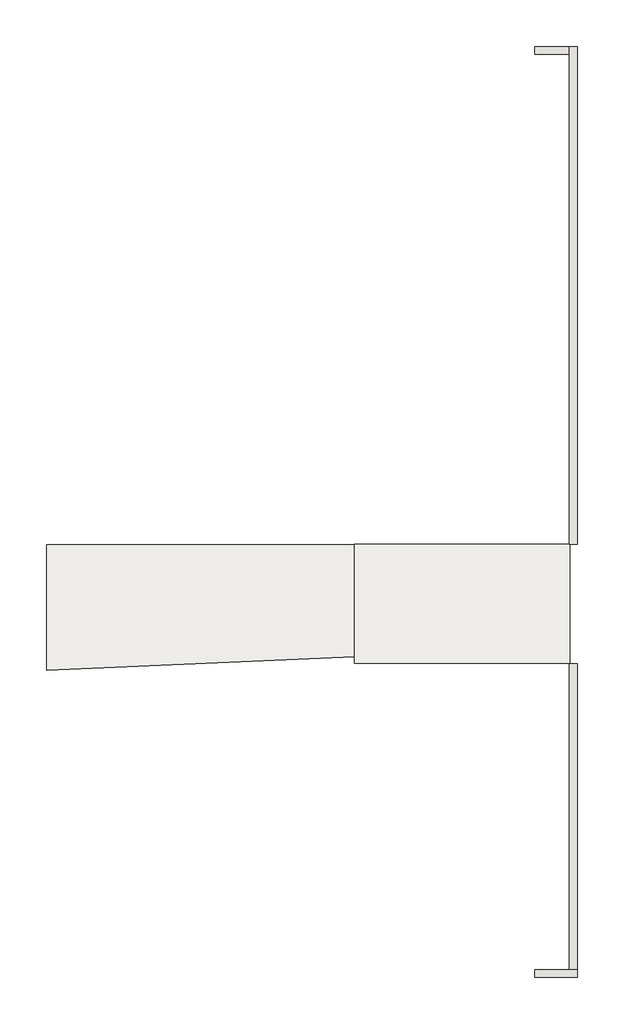
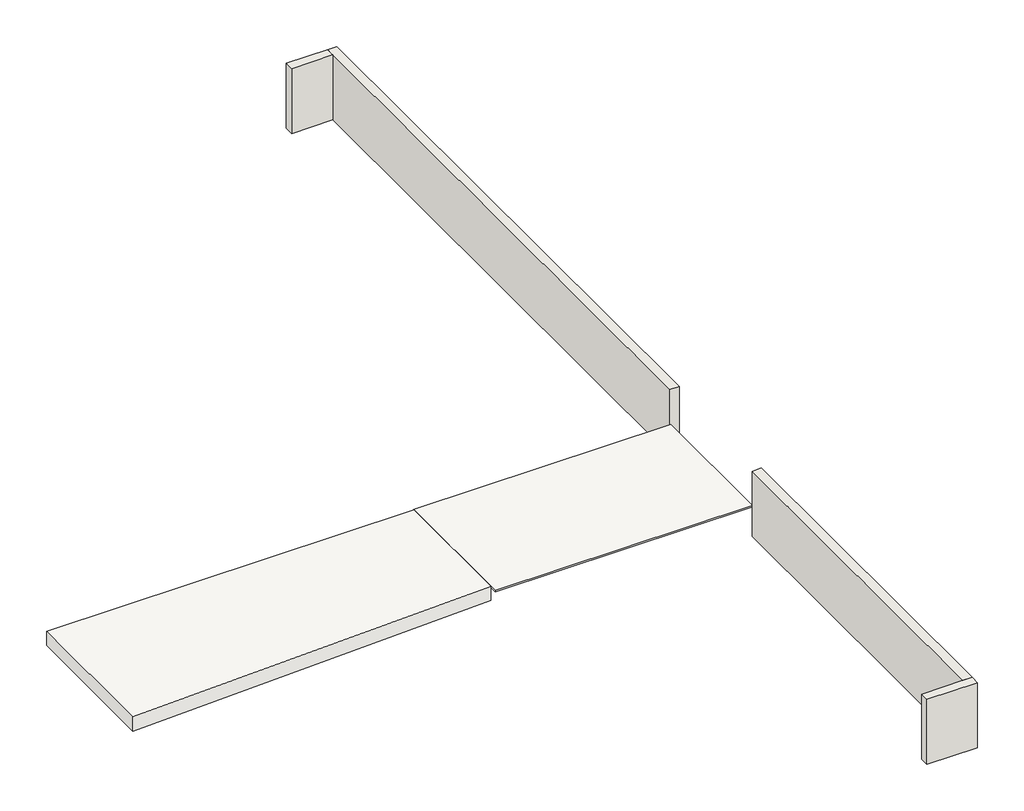
# One storey: 4 walls, 2 slabs.
"""IFC4 building model written with IfcOpenShell, lengths in millimetres."""

from ifc_helpers import new_model, si_unit, frame, origin, place, context, project, spatial, polyline, outline, extrude, faceted_brep, element, save

model = new_model("IFC4")

# Units and contexts
model_context = context("Model", 3, world=origin())
ifc_project = project(units=[si_unit("LENGTHUNIT", "METRE", prefix="MILLI")], contexts=[model_context])

# Site, building, storey
site = spatial("IfcSite", under=ifc_project)
building = spatial("IfcBuilding", under=site)
storey = spatial("IfcBuildingStorey", under=building, Name="otopark", Elevation=-660.0)

# Slabs
placement = place(None, origin())
element("IfcSlab", 1, ObjectType="aa Taban 3 cm beyaz mermer", at=placement, inside=storey, context=model_context, shape_type="SweptSolid", body=[
    extrude(outline(polyline([(11307.8247381, -10362.4985309), (11307.8247381, -7282.4985309), (16907.8247381, -7282.4985309), (16907.8247381, -10362.4985309), (11307.8247381, -10362.4985309)])), frame((0.0, 0.0, -689.8), z_axis=(0.0, 0.0, 1.0), x_axis=(1.0, 0.0, 0.0)), (0.0, 0.0, 1.0), 30.0),
])
element("IfcSlab", 2, ObjectType="15mm Foundation Slab", at=placement, inside=storey, context=model_context, shape_type="Brep", body=[
    faceted_brep([(11307.8247381, -7292.4985309, -989.8), (11307.8247381, -10202.8108149, -989.8), (3307.8247381, -10546.9586554, -989.8), (3307.8247381, -7292.4985309, -989.8), (11307.8247381, -7292.4985309, -659.8), (3307.8247381, -7292.4985309, -659.8), (3307.8247381, -10546.9586554, -659.8), (11307.8247381, -10202.8108149, -659.8), (3307.8247381, -7292.4985309, -930.0)], [[[0, 1, 2, 3]], [[4, 5, 6, 7]], [[1, 0, 4, 7]], [[2, 1, 7, 6]], [[3, 2, 6, 5, 8]], [[0, 3, 8, 5, 4]]]),
])

# Walls
element("IfcWall", 3, ObjectType="Generic - 200mm - Filled", at=placement, inside=storey, context=model_context, shape_type="SweptSolid", body=[
    extrude(outline(polyline([(17100.9898032, -10378.1142076), (17100.9898032, -18328.1142076), (16900.9898032, -18328.1142076), (16900.9898032, -10378.1142076), (17100.9898032, -10378.1142076)])), frame((0.0, 0.0, -1360.0), z_axis=(0.0, 0.0, 1.0), x_axis=(1.0, 0.0, 0.0)), (0.0, 0.0, 1.0), 1500.0),
])
element("IfcWall", 4, ObjectType="Generic - 200mm - Filled", at=placement, inside=storey, context=model_context, shape_type="Brep", body=[
    faceted_brep([(17100.9898032, -7272.9665452, -1360.0), (17100.9898032, 5647.0334548, -1360.0), (17100.9898032, 5647.0334548, 140.0), (17100.9898032, -7272.9665452, 140.0), (16900.9898032, -7272.9665452, -1360.0), (16900.9898032, -7272.9665452, 140.0), (16900.9898032, 5447.0334548, 140.0), (16900.9898032, 5647.0334548, 140.0), (16900.9898032, 5647.0334548, -1360.0), (16900.9898032, 5447.0334548, -1360.0)], [[[0, 1, 2, 3]], [[4, 5, 6, 7, 8, 9]], [[1, 0, 4, 9, 8]], [[3, 2, 7, 6, 5]], [[0, 3, 5, 4]], [[2, 1, 8, 7]]]),
])
element("IfcWall", 5, ObjectType="Generic - 200mm - Filled", at=placement, inside=storey, context=model_context, shape_type="Brep", body=[
    faceted_brep([(17100.9898032, -18328.1142076, -1360.0), (16900.9898032, -18328.1142076, -1360.0), (16000.9898032, -18328.1142076, -1360.0), (16000.9898032, -18328.1142076, 140.0), (16900.9898032, -18328.1142076, 140.0), (17100.9898032, -18328.1142076, 140.0), (17100.9898032, -18528.1142076, -1360.0), (17100.9898032, -18528.1142076, 140.0), (16000.9898032, -18528.1142076, 140.0), (16000.9898032, -18528.1142076, -1360.0)], [[[0, 1, 2, 3, 4, 5]], [[6, 7, 8, 9]], [[2, 1, 0, 6, 9]], [[3, 2, 9, 8]], [[5, 4, 3, 8, 7]], [[0, 5, 7, 6]]]),
])
element("IfcWall", 6, ObjectType="Generic - 200mm - Filled", at=placement, inside=storey, context=model_context, shape_type="SweptSolid", body=[
    extrude(outline(polyline([(16000.9898032, 5647.0334548), (16900.9898032, 5647.0334548), (16900.9898032, 5447.0334548), (16000.9898032, 5447.0334548), (16000.9898032, 5647.0334548)])), frame((0.0, 0.0, -1360.0), z_axis=(0.0, 0.0, 1.0), x_axis=(1.0, 0.0, 0.0)), (0.0, 0.0, 1.0), 1500.0),
])

save(model, "model.ifc")

# Revit data of these elements
# Project information
#   Project Issue Date = "Issue Date"
#   Project Status = "Project Status"
#   Client Name = "Owner"
#   Project Address = "Enter address here"
#   Project Name = "Project Name"
#   Project Number = "0001"
# Type "aa Taban 3 cm beyaz mermer"
#   Function = 0
#   Layers, outside or top first: 3 cm "Stone" (function 1)
# Type "15mm Foundation Slab"
#   Layers, outside or top first: 3 cm "Travertine" (function 1); 30 cm "Concrete, Cast In Situ" (function 1)
# Type "Generic - 200mm - Filled"
#   Layers, outside or top first: 20 cm no material (function 1)
# Element 1 (IfcSlab, "aa Taban 3 cm beyaz mermer")
#   Height Offset From Level = 0.02 cm
#   Phase Created = Phase 1
#   Materials on its faces: "Stone"
# Element 2 (IfcSlab, "15mm Foundation Slab")
#   Height Offset From Level = 0.02 cm
#   built-in parameter 1001954 = 1
#   Phase Created = Phase 1
#   Materials on its faces: "Concrete, Cast In Situ", "Travertine"
# Elements 3, 4, 5, 6 (IfcWall, "Generic - 200mm - Filled")
#   built-in parameter 1001111 = -70 cm
#   Top Offset = 0 cm
#   Base Offset = -70 cm
#   Unconnected Height = 150 cm
#   wall height = 150 cm
#   Phase Created = Phase 1
#   Base Constraint = otopark
#   Materials on its faces: "Default Wall"
# Materials
#   "Stone": class "Stone", colour RGB 120 120 120, transparency 0, Description = "Stone, rough tan", Cost = 0
#   "Travertine": class "Stone", colour RGB 120 120 120, transparency 0, Description = "Travertine, cream, matte", Cost = 0
#   "Concrete, Cast In Situ": class "Concrete", colour RGB 192 192 192, transparency 0, Description = "physical material", Cost = 0
#   "Default Wall": class "Miscellaneous", colour RGB 128 128 128, transparency 0, Cost = 0
